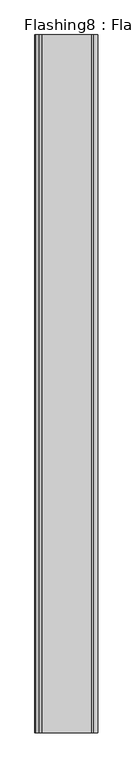
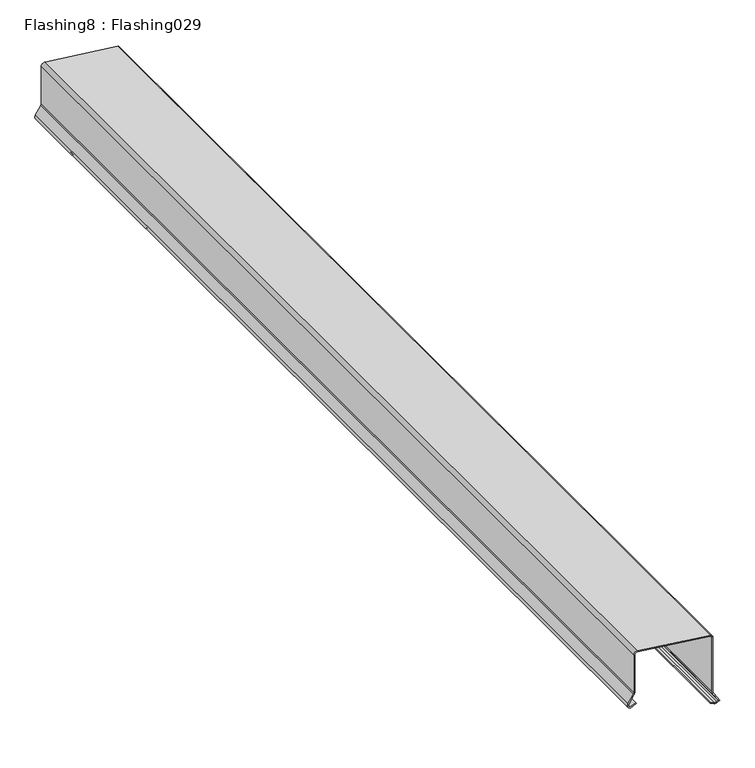
"""IFC4 building model written with IfcOpenShell, lengths in millimetres: proxy geometry, Flashing8 : Flashing029."""

from ifc_helpers import new_model, si_unit, point, frame, frame_2d, origin, place, context, project, spatial, polyline, circle_curve, trimmed, segment, composite_curve, outline, extrude, source, transform, mapped, element, save


def flashing8_flashing029_23744907(model_context):
    return source(origin(), model_context, "Body", "SweptSolid", [
        extrude(outline(composite_curve([segment(polyline([(40086.398437, -7266.956055), (40092.152344, -7255.346191), (40093.9490864, -7256.2366656), (40088.6846745, -7266.8588577), (40089.8466166, -7268.7750305)]), True, "CONTINUOUS"), segment(trimmed(circle_curve(frame_2d((40093.4434175, -7266.287785)), 4.3730273), [point((40089.8466166, -7268.7750305))], [point((40095.7266973, -7270.0173964))], True, "CARTESIAN"), True, "CONTINUOUS"), segment(polyline([(40095.7266973, -7270.0173964), (40111.7309891, -7259.7605083)]), True, "CONTINUOUS"), segment(trimmed(circle_curve(frame_2d((40115.861873, -7265.806759)), 7.32266), [point((40111.7309891, -7259.7605083))], [point((40116.1385872, -7258.4893292))], False, "CARTESIAN"), True, "CONTINUOUS"), segment(polyline([(40116.1385872, -7258.4893292), (40193.276665, -7258.4893292)]), True, "CONTINUOUS"), segment(trimmed(circle_curve(frame_2d((40193.367253, -7254.1255777)), 4.3646917), [point((40193.276665, -7258.4893292))], [point((40197.6973721, -7253.5773062))], True, "CARTESIAN"), True, "CONTINUOUS"), segment(polyline([(40197.6973721, -7253.5773062), (40180.4916036, -7111.7967854)]), True, "CONTINUOUS"), segment(trimmed(circle_curve(frame_2d((40175.841451, -7112.759368)), 4.7487351), [point((40180.4916036, -7111.7967854))], [point((40175.9416385, -7108.0116899))], True, "CARTESIAN"), True, "CONTINUOUS"), segment(polyline([(40175.9416385, -7108.0116899), (40064.0437764, -7108.0116899)]), True, "CONTINUOUS"), segment(trimmed(circle_curve(frame_2d((40064.0983061, -7099.1269875)), 8.8848697), [point((40064.0437764, -7108.0116899))], [point((40059.2697952, -7106.5852979))], False, "CARTESIAN"), True, "CONTINUOUS"), segment(polyline([(40059.2697952, -7106.5852979), (40042.6162498, -7095.8037908), (40040.6845786, -7098.9401191)]), True, "CONTINUOUS"), segment(trimmed(circle_curve(frame_2d((40044.441402, -7101.272247)), 4.4218257), [point((40040.6845786, -7098.9401191))], [point((40040.4164008, -7103.1030686))], True, "CARTESIAN"), True, "CONTINUOUS"), segment(polyline([(40040.4164008, -7103.1030686), (40043.7762965, -7110.0176247), (40041.972656, -7110.894043), (40038.6026561, -7103.9586928)]), True, "CONTINUOUS"), segment(trimmed(circle_curve(frame_2d((40044.441402, -7101.272247)), 6.4271257), [point((40038.6026561, -7103.9586928))], [point((40038.9788223, -7097.8857786))], False, "CARTESIAN"), True, "CONTINUOUS"), segment(polyline([(40038.9788223, -7097.8857786), (40041.984375, -7093.005859), (40060.3595819, -7104.9019699)]), True, "CONTINUOUS"), segment(trimmed(circle_curve(frame_2d((40064.0983061, -7099.1269875)), 6.8795697), [point((40060.3595819, -7104.9019699))], [point((40064.0503229, -7106.0063899))], True, "CARTESIAN"), True, "CONTINUOUS"), segment(polyline([(40064.0503229, -7106.0063899), (40175.960936, -7106.0063899)]), True, "CONTINUOUS"), segment(trimmed(circle_curve(frame_2d((40175.841451, -7112.759368)), 6.7540351), [point((40175.960936, -7106.0063899))], [point((40182.4731108, -7111.4794937))], False, "CARTESIAN"), True, "CONTINUOUS"), segment(polyline([(40182.4731108, -7111.4794937), (40199.6874998, -7253.3310503)]), True, "CONTINUOUS"), segment(trimmed(circle_curve(frame_2d((40193.367253, -7254.1255777)), 6.3699917), [point((40199.6874998, -7253.3310503))], [point((40193.2578143, -7260.4946292))], False, "CARTESIAN"), True, "CONTINUOUS"), segment(polyline([(40193.2578143, -7260.4946292), (40116.0976578, -7260.4946292)]), True, "CONTINUOUS"), segment(trimmed(circle_curve(frame_2d((40115.861873, -7265.806759)), 5.31736), [point((40116.0976578, -7260.4946292))], [point((40112.8398424, -7261.4316421))], True, "CARTESIAN"), True, "CONTINUOUS"), segment(polyline([(40112.8398424, -7261.4316421), (40096.7929689, -7271.7158201)]), True, "CONTINUOUS"), segment(trimmed(circle_curve(frame_2d((40093.4434175, -7266.287785)), 6.3783273), [point((40096.7929689, -7271.7158201))], [point((40088.1601567, -7269.8613287))], False, "CARTESIAN"), True, "CONTINUOUS"), segment(polyline([(40088.1601567, -7269.8613287), (40086.398437, -7266.956055)]), True, "CONTINUOUS")], self_intersect=False)), frame((0.0, 7982.1531721, 0.0), z_axis=(0.0, 1.0, 0.0), x_axis=(0.0, 0.0, 1.0)), (0.0, 0.0, 1.0), 1999.85),
    ])


if __name__ == "__main__":
    model = new_model("IFC4")
    model_context = context("Model", 3, world=origin())
    ifc_project = project(units=[si_unit("LENGTHUNIT", "METRE", prefix="MILLI")], contexts=[model_context])
    site = spatial("IfcSite", under=ifc_project)
    building = spatial("IfcBuilding", under=site)
    placement = place(None, origin())
    flashing8_flashing029_shape = flashing8_flashing029_23744907(model_context)
    element("IfcBuildingElementProxy", 1, Name="Flashing8 : Flashing029", ObjectType="Flashing8 : Flashing029", at=placement, inside=building, context=model_context, shape_type="MappedRepresentation", body=[
        mapped(flashing8_flashing029_shape, transform((0.0, 0.0, 0.0), x_axis=(1.0, 0.0, 0.0), y_axis=(0.0, 1.0, 0.0), z_axis=(0.0, 0.0, 1.0))),
    ])
    save(model, "model.ifc")

# Revit data of these elements
# Type "Flashing8 : Flashing029"
#   NameOverride = "Flashing029"
# Element 1 (IfcBuildingElementProxy, "Flashing8 : Flashing029")
#   Materials on its faces: "METAL COPING"
# Materials
#   "METAL COPING": class "Unassigned", colour RGB 128 128 128, transparency 0
